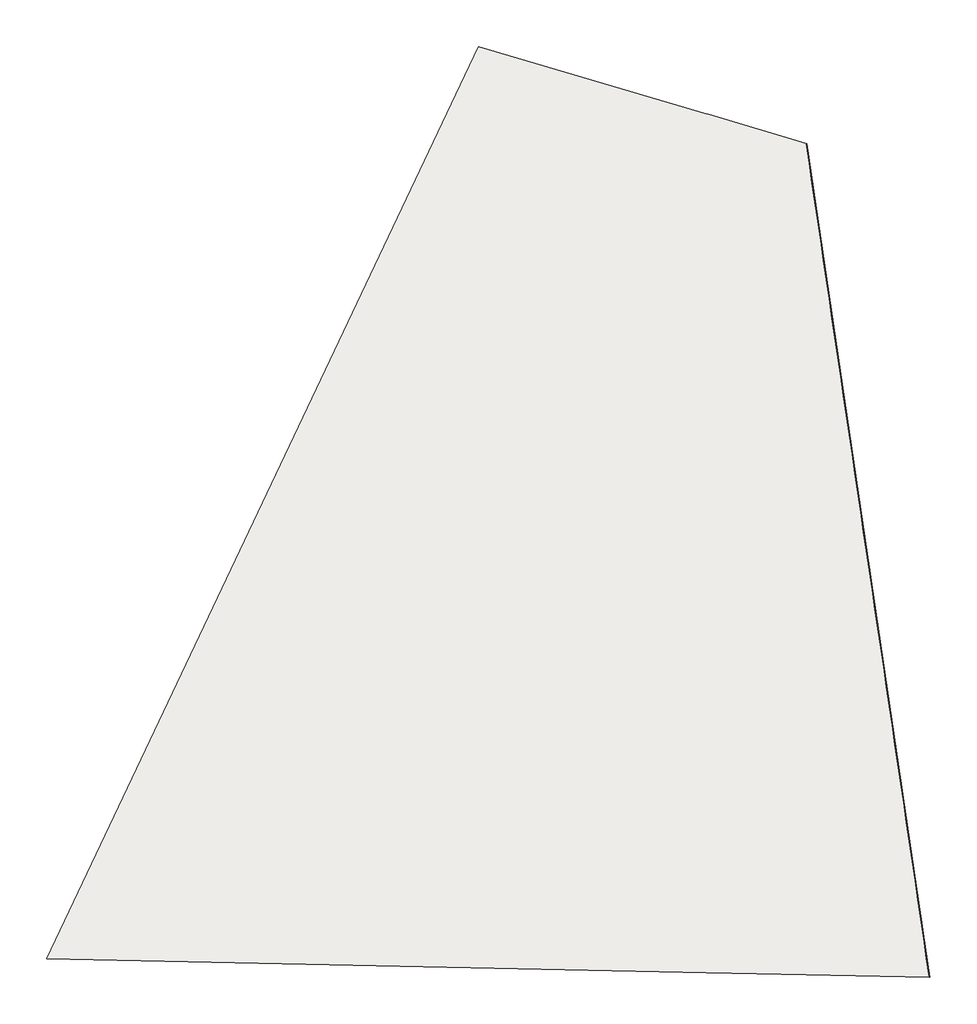
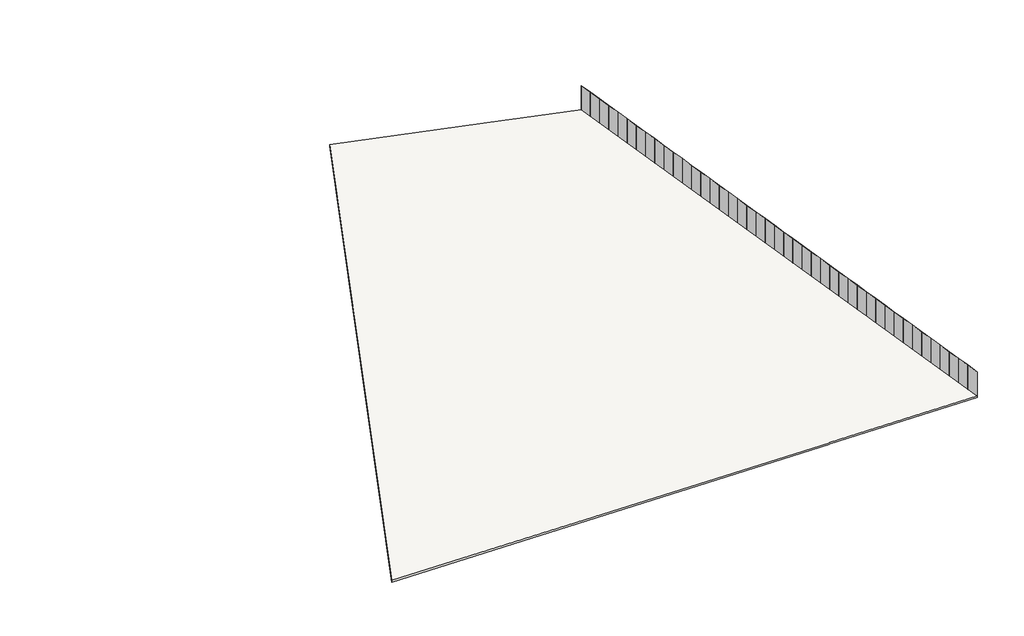
# One storey: 44 plates, 1 slab.
"""IFC4 building model written with IfcOpenShell, lengths in millimetres."""

import ifcopenshell
import ifcopenshell.guid

model = None  # the IFC model being written
_history = None  # IfcOwnerHistory: only IFC2X3 demands one
_inside = {}  # id of a spatial element -> (the spatial element, [elements in it])
_under = {}  # id of a project, library or spatial element -> (it, [spatial elements below it])
_declared = {}  # id of a project -> (the project, [libraries it declares])
_typed = {}  # id of a type object -> (the type object, [elements of that type])
_made_of = {}  # id of a material, layer set ... -> (it, [elements and type objects made of it])


def new_model(schema):
    """Start an empty IFC model of exactly this schema.

    Asked for "IFC4X3", IfcOpenShell would pick the latest addendum, in which some entities
    have other attributes; the version numbers below select the first issue.
    IFC2X3 requires an IfcOwnerHistory on every rooted entity: one is made here for all.
    """
    global model, _history
    if schema == "IFC4X3":
        model = ifcopenshell.file(schema_version=(4, 3, 0, 0))
    else:
        model = ifcopenshell.file(schema=schema)
    _inside.clear()
    _under.clear()
    _declared.clear()
    _typed.clear()
    _made_of.clear()
    _history = None
    if model.schema == "IFC2X3":
        org = make("IfcOrganization", Name="unknown")
        user = make(
            "IfcPersonAndOrganization",
            ThePerson=make("IfcPerson", FamilyName="unknown"),
            TheOrganization=org,
        )
        app = make(
            "IfcApplication",
            ApplicationDeveloper=org,
            Version="unknown",
            ApplicationFullName="unknown",
            ApplicationIdentifier="unknown",
        )
        _history = make(
            "IfcOwnerHistory",
            OwningUser=user,
            OwningApplication=app,
            ChangeAction="ADDED",
            CreationDate=0,
        )
    return model


def make(cls, **values):
    """One entity of the class cls with the attributes given. An attribute that is None is left unset."""
    return model.create_entity(
        cls, **{name: value for name, value in values.items() if value is not None}
    )


def rooted(cls, **values):
    """An entity with a GlobalId (a new one), such as an element, a storey or a relation."""
    return make(cls, GlobalId=ifcopenshell.guid.new(), OwnerHistory=_history, **values)


def si_unit(unit_type, name, prefix=None):
    """IfcSIUnit, for example si_unit("LENGTHUNIT", "METRE", prefix="MILLI")."""
    return make("IfcSIUnit", UnitType=unit_type, Prefix=prefix, Name=name)


def assignment(units):
    """IfcUnitAssignment: the units of a project."""
    return None if units is None else make("IfcUnitAssignment", Units=units)


def point(xyz):
    """IfcCartesianPoint."""
    return None if xyz is None else make("IfcCartesianPoint", Coordinates=xyz)


def direction(xyz):
    """IfcDirection."""
    return None if xyz is None else make("IfcDirection", DirectionRatios=xyz)


def frame(location, z_axis=None, x_axis=None):
    """IfcAxis2Placement3D, a coordinate frame: its origin and axes. An axis left out is left unset."""
    return make(
        "IfcAxis2Placement3D",
        Location=point(location),
        Axis=direction(z_axis),
        RefDirection=direction(x_axis),
    )


def origin():
    """The frame at (0, 0, 0) with its axes left unset."""
    return frame((0.0, 0.0, 0.0))


def origin_with_axes():
    """The frame at (0, 0, 0) with the z axis (0, 0, 1) and the x axis (1, 0, 0) written out."""
    return frame((0.0, 0.0, 0.0), z_axis=(0.0, 0.0, 1.0), x_axis=(1.0, 0.0, 0.0))


def place(relative_to, where):
    """IfcLocalPlacement: puts the frame where relative to a parent placement (None: the world)."""
    return make(
        "IfcLocalPlacement", PlacementRelTo=relative_to, RelativePlacement=where
    )


def context(
    kind, dimensions, precision=None, world=None, true_north=None, identifier=None
):
    """IfcGeometricRepresentationContext, for example the 3D "Model" context."""
    return make(
        "IfcGeometricRepresentationContext",
        ContextIdentifier=identifier,
        ContextType=kind,
        CoordinateSpaceDimension=dimensions,
        Precision=precision,
        WorldCoordinateSystem=world,
        TrueNorth=true_north,
    )


def project(units=None, contexts=None):
    """IfcProject with its units and contexts."""
    return rooted(
        "IfcProject",
        Name="project",
        RepresentationContexts=contexts,
        UnitsInContext=assignment(units),
    )


def spatial(cls, under=None, at=None, **own):
    """A site, building, storey or space (cls), placed at a placement, below another one or the project."""
    s = rooted(cls, ObjectPlacement=at, **own)
    if under is not None:
        _under.setdefault(under.id(), (under, []))[1].append(s)
    return s


def polyline(points):
    """IfcPolyline through the points."""
    return make("IfcPolyline", Points=[point(p) for p in points])


def outline(outer, holes=None, kind="AREA"):
    """IfcArbitraryClosedProfileDef: a profile drawn as a closed curve; with holes, ...WithVoids."""
    if holes is None:
        return make("IfcArbitraryClosedProfileDef", ProfileType=kind, OuterCurve=outer)
    return make(
        "IfcArbitraryProfileDefWithVoids",
        ProfileType=kind,
        OuterCurve=outer,
        InnerCurves=holes,
    )


def extrude(swept, where, along, depth):
    """IfcExtrudedAreaSolid: the profile swept, set in the frame where, extruded along a direction by depth."""
    return make(
        "IfcExtrudedAreaSolid",
        SweptArea=swept,
        Position=where,
        ExtrudedDirection=direction(along),
        Depth=depth,
    )


def faces_of(points, faces, orient=None, outer=None):
    """IfcFace entities. A face is a list of loops; a loop is a list of indices into points, from 0.

    orient and outer hold one flag for each loop. By default every Orientation is true, the
    first loop of a face is its IfcFaceOuterBound and the others are IfcFaceBound.
    """
    made = []
    for i, loops in enumerate(faces):
        bounds = []
        for j, loop in enumerate(loops):
            is_outer = j == 0 if outer is None else outer[i][j]
            bounds.append(
                make(
                    "IfcFaceOuterBound" if is_outer else "IfcFaceBound",
                    Bound=make("IfcPolyLoop", Polygon=[points[k] for k in loop]),
                    Orientation=True if orient is None else orient[i][j],
                )
            )
        made.append(make("IfcFace", Bounds=bounds))
    return made


def faceted_brep(points, faces, orient=None, outer=None, voids=None):
    """IfcFacetedBrep: a solid bounded by flat faces; with voids (closed shells), ...WithVoids."""
    shared = [point(p) for p in points]
    hull = make("IfcClosedShell", CfsFaces=faces_of(shared, faces, orient, outer))
    if voids is None:
        return make("IfcFacetedBrep", Outer=hull)
    return make(
        "IfcFacetedBrepWithVoids",
        Outer=hull,
        Voids=[
            make(cls, CfsFaces=faces_of(shared, fs, o, b)) for cls, fs, o, b in voids
        ],
    )


def shape(context_of_items, identifier, shape_type, items):
    """IfcShapeRepresentation: the items that make up one representation, for example the "Body"."""
    return make(
        "IfcShapeRepresentation",
        ContextOfItems=context_of_items,
        RepresentationIdentifier=identifier,
        RepresentationType=shape_type,
        Items=items,
    )


def source(mapping_origin, context_of_items, identifier, shape_type, items):
    """IfcRepresentationMap: a shape defined once, which mapped items show again and again."""
    return make(
        "IfcRepresentationMap",
        MappingOrigin=mapping_origin,
        MappedRepresentation=shape(context_of_items, identifier, shape_type, items),
    )


def transform(
    local_origin,
    x_axis=None,
    y_axis=None,
    z_axis=None,
    scale=None,
    scale2=None,
    scale3=None,
    uniform=True,
):
    """IfcCartesianTransformationOperator3D, or its non-uniform kind. x_axis, y_axis, z_axis: its Axis1, 2, 3."""
    if uniform:
        return make(
            "IfcCartesianTransformationOperator3D",
            Axis1=direction(x_axis),
            Axis2=direction(y_axis),
            LocalOrigin=point(local_origin),
            Scale=scale,
            Axis3=direction(z_axis),
        )
    return make(
        "IfcCartesianTransformationOperator3DnonUniform",
        Axis1=direction(x_axis),
        Axis2=direction(y_axis),
        LocalOrigin=point(local_origin),
        Scale=scale,
        Axis3=direction(z_axis),
        Scale2=scale2,
        Scale3=scale3,
    )


def mapped(mapping_source, mapping_target):
    """IfcMappedItem: shows the shape of a source again, moved by a transform."""
    return make(
        "IfcMappedItem", MappingSource=mapping_source, MappingTarget=mapping_target
    )


def made_of(thing, what):
    """Note that an element or type object is made of a material, layer set ...; save() writes the relation."""
    if what is not None:
        _made_of.setdefault(what.id(), (what, []))[1].append(thing)
    return thing


def element(
    cls,
    number,
    at=None,
    inside=None,
    cuts=None,
    type_object=None,
    material=None,
    context=None,
    identifier="Body",
    shape_type=None,
    held_by="IfcProductDefinitionShape",
    body=None,
    shapes=None,
    **own,
):
    """One element of the class cls, such as IfcWall. Its Tag is "e" and its number.

    at: its placement. inside: the storey or other place that contains it. cuts: it is an
    opening in that element (IfcRelVoidsElement). A single representation is given by context,
    identifier, shape_type and body (its items); several are given by shapes. held_by: the class
    of the entity that holds the representations. save() writes the other relations.
    """
    e = rooted(cls, Tag="e%d" % number, ObjectPlacement=at, **own)
    if body is not None:
        shapes = [shape(context, identifier, shape_type, body)]
    if shapes is not None:
        e.Representation = make(held_by, Representations=shapes)
    if inside is not None:
        _inside.setdefault(inside.id(), (inside, []))[1].append(e)
    if cuts is not None:
        rooted(
            "IfcRelVoidsElement", RelatingBuildingElement=cuts, RelatedOpeningElement=e
        )
    if type_object is not None:
        _typed.setdefault(type_object.id(), (type_object, []))[1].append(e)
    return made_of(e, material)


def aggregate(whole, parts):
    """IfcRelAggregates: a whole, such as a stair, and the parts it consists of."""
    return rooted("IfcRelAggregates", RelatingObject=whole, RelatedObjects=parts)


def save(model, path):
    """Write the relations noted so far, then the file.

    IfcRelAggregates (storeys below a building ...), IfcRelContainedInSpatialStructure (elements
    in a storey), IfcRelDefinesByType, IfcRelAssociatesMaterial and IfcRelDeclares: one each for
    every whole, place, type object, material and project.
    """
    for whole, parts in _under.values():
        aggregate(whole, parts)
    for where, things in _inside.values():
        rooted(
            "IfcRelContainedInSpatialStructure",
            RelatedElements=things,
            RelatingStructure=where,
        )
    for kind, things in _typed.values():
        rooted("IfcRelDefinesByType", RelatedObjects=things, RelatingType=kind)
    for what, things in _made_of.values():
        rooted("IfcRelAssociatesMaterial", RelatedObjects=things, RelatingMaterial=what)
    for by, libraries in _declared.values():
        rooted("IfcRelDeclares", RelatingContext=by, RelatedDefinitions=libraries)
    model.write(path)


def painel_do_sistema_b8becc76(model_context):
    return source(origin(), model_context, "Body", "SweptSolid", [
        extrude(outline(polyline([(1499.9999925, 24.5), (-1499.9999925, 24.5), (-1499.9999925, 49.5), (1499.9999925, 49.5), (1499.9999925, 24.5)])), origin_with_axes(), (0.0, 0.0, 1.0), 1500.0),
    ])


def painel_do_sistema_42adfd5d(model_context):
    return source(origin(), model_context, "Body", "SweptSolid", [
        extrude(outline(polyline([(1499.9999925, 24.5), (-1499.9999925, 24.5), (-1499.9999925, 49.5), (1499.9999925, 49.5), (1499.9999925, 24.5)])), origin_with_axes(), (0.0, 0.0, 1.0), 20.0931032),
    ])


model = new_model("IFC4")

# Units and contexts
model_context = context("Model", 3, world=origin())
ifc_project = project(units=[si_unit("LENGTHUNIT", "METRE", prefix="MILLI")], contexts=[model_context])

# Site, building, storey
site = spatial("IfcSite", under=ifc_project)
building = spatial("IfcBuilding", under=site)
storey = spatial("IfcBuildingStorey", under=building, Name="Nível 9", Elevation=12000.0)

# Plates
placement = place(None, origin())
painel_do_sistema_shape = painel_do_sistema_b8becc76(model_context)
element("IfcPlate", 1, ObjectType="Painel do sistema : Envidraçado", at=placement, inside=storey, context=model_context, shape_type="MappedRepresentation", body=[
    mapped(painel_do_sistema_shape, transform((27835.0106579, -36774.1442579, 13500.0000075), x_axis=(0.0, 0.0, 1.0), y_axis=(-0.9892699032546327, -0.1460994815684493, 0.0), z_axis=(0.1460994815684493, -0.9892699032546327, 0.0))),
])
element("IfcPlate", 2, ObjectType="Painel do sistema : Envidraçado", at=placement, inside=storey, context=model_context, shape_type="MappedRepresentation", body=[
    mapped(painel_do_sistema_shape, transform((27615.8614356, -35290.239403, 13500.0000075), x_axis=(0.0, 0.0, 1.0), y_axis=(-0.9892699032546328, -0.1460994815684489, 0.0), z_axis=(0.1460994815684489, -0.9892699032546328, 0.0))),
])
element("IfcPlate", 3, ObjectType="Painel do sistema : Envidraçado", at=placement, inside=storey, context=model_context, shape_type="MappedRepresentation", body=[
    mapped(painel_do_sistema_shape, transform((27396.7122132, -33806.3345481, 13500.0000075), x_axis=(0.0, 0.0, 1.0), y_axis=(-0.9892699032546323, -0.14609948156845212, 0.0), z_axis=(0.14609948156845212, -0.9892699032546323, 0.0))),
])
element("IfcPlate", 4, ObjectType="Painel do sistema : Envidraçado", at=placement, inside=storey, context=model_context, shape_type="MappedRepresentation", body=[
    mapped(painel_do_sistema_shape, transform((27177.5629909, -32322.4296932, 13500.0000075), x_axis=(0.0, 0.0, 1.0), y_axis=(-0.9892699032546327, -0.1460994815684493, 0.0), z_axis=(0.1460994815684493, -0.9892699032546327, 0.0))),
])
element("IfcPlate", 5, ObjectType="Painel do sistema : Envidraçado", at=placement, inside=storey, context=model_context, shape_type="MappedRepresentation", body=[
    mapped(painel_do_sistema_shape, transform((26958.4137685, -30838.5248383, 13500.0000075), x_axis=(0.0, 0.0, 1.0), y_axis=(-0.9892699032546327, -0.1460994815684493, 0.0), z_axis=(0.1460994815684493, -0.9892699032546327, 0.0))),
])
element("IfcPlate", 6, ObjectType="Painel do sistema : Envidraçado", at=placement, inside=storey, context=model_context, shape_type="MappedRepresentation", body=[
    mapped(painel_do_sistema_shape, transform((26739.2645462, -29354.6199835, 13500.0000075), x_axis=(0.0, 0.0, 1.0), y_axis=(-0.9892699032546327, -0.1460994815684493, 0.0), z_axis=(0.1460994815684493, -0.9892699032546327, 0.0))),
])
element("IfcPlate", 7, ObjectType="Painel do sistema : Envidraçado", at=placement, inside=storey, context=model_context, shape_type="MappedRepresentation", body=[
    mapped(painel_do_sistema_shape, transform((26520.1153238, -27870.7151286, 13500.0000075), x_axis=(0.0, 0.0, 1.0), y_axis=(-0.9892699032546324, -0.14609948156845168, 0.0), z_axis=(0.14609948156845168, -0.9892699032546324, 0.0))),
])
element("IfcPlate", 8, ObjectType="Painel do sistema : Envidraçado", at=placement, inside=storey, context=model_context, shape_type="MappedRepresentation", body=[
    mapped(painel_do_sistema_shape, transform((26300.9661014, -26386.8102737, 13500.0000075), x_axis=(0.0, 0.0, 1.0), y_axis=(-0.9892699032546327, -0.1460994815684493, 0.0), z_axis=(0.1460994815684493, -0.9892699032546327, 0.0))),
])
element("IfcPlate", 9, ObjectType="Painel do sistema : Envidraçado", at=placement, inside=storey, context=model_context, shape_type="MappedRepresentation", body=[
    mapped(painel_do_sistema_shape, transform((26081.8168791, -24902.9054188, 13500.0000075), x_axis=(0.0, 0.0, 1.0), y_axis=(-0.9892699032546328, -0.1460994815684489, 0.0), z_axis=(0.1460994815684489, -0.9892699032546328, 0.0))),
])
element("IfcPlate", 10, ObjectType="Painel do sistema : Envidraçado", at=placement, inside=storey, context=model_context, shape_type="MappedRepresentation", body=[
    mapped(painel_do_sistema_shape, transform((25862.6676567, -23419.0005639, 13500.0000075), x_axis=(0.0, 0.0, 1.0), y_axis=(-0.9892699032546324, -0.14609948156845168, 0.0), z_axis=(0.14609948156845168, -0.9892699032546324, 0.0))),
])
element("IfcPlate", 11, ObjectType="Painel do sistema : Envidraçado", at=placement, inside=storey, context=model_context, shape_type="MappedRepresentation", body=[
    mapped(painel_do_sistema_shape, transform((25643.5184344, -21935.095709, 13500.0000075), x_axis=(0.0, 0.0, 1.0), y_axis=(-0.9892699032546327, -0.1460994815684493, 0.0), z_axis=(0.1460994815684493, -0.9892699032546327, 0.0))),
])
element("IfcPlate", 12, ObjectType="Painel do sistema : Envidraçado", at=placement, inside=storey, context=model_context, shape_type="MappedRepresentation", body=[
    mapped(painel_do_sistema_shape, transform((25424.369212, -20451.1908542, 13500.0000075), x_axis=(0.0, 0.0, 1.0), y_axis=(-0.9892699032546324, -0.14609948156845168, 0.0), z_axis=(0.14609948156845168, -0.9892699032546324, 0.0))),
])
element("IfcPlate", 13, ObjectType="Painel do sistema : Envidraçado", at=placement, inside=storey, context=model_context, shape_type="MappedRepresentation", body=[
    mapped(painel_do_sistema_shape, transform((25205.2199897, -18967.2859993, 13500.0000075), x_axis=(0.0, 0.0, 1.0), y_axis=(-0.9892699032546328, -0.14609948156844865, 0.0), z_axis=(0.14609948156844865, -0.9892699032546328, 0.0))),
])
element("IfcPlate", 14, ObjectType="Painel do sistema : Envidraçado", at=placement, inside=storey, context=model_context, shape_type="MappedRepresentation", body=[
    mapped(painel_do_sistema_shape, transform((24986.0707673, -17483.3811444, 13500.0000075), x_axis=(0.0, 0.0, 1.0), y_axis=(-0.9892699032546328, -0.1460994815684491, 0.0), z_axis=(0.1460994815684491, -0.9892699032546328, 0.0))),
])
element("IfcPlate", 15, ObjectType="Painel do sistema : Envidraçado", at=placement, inside=storey, context=model_context, shape_type="MappedRepresentation", body=[
    mapped(painel_do_sistema_shape, transform((24766.921545, -15999.4762895, 13500.0000075), x_axis=(0.0, 0.0, 1.0), y_axis=(-0.9892699032546327, -0.1460994815684493, 0.0), z_axis=(0.1460994815684493, -0.9892699032546327, 0.0))),
])
element("IfcPlate", 16, ObjectType="Painel do sistema : Envidraçado", at=placement, inside=storey, context=model_context, shape_type="MappedRepresentation", body=[
    mapped(painel_do_sistema_shape, transform((24547.7723226, -14515.5714346, 13500.0000075), x_axis=(0.0, 0.0, 1.0), y_axis=(-0.9892699032546324, -0.14609948156845168, 0.0), z_axis=(0.14609948156845168, -0.9892699032546324, 0.0))),
])
element("IfcPlate", 17, ObjectType="Painel do sistema : Envidraçado", at=placement, inside=storey, context=model_context, shape_type="MappedRepresentation", body=[
    mapped(painel_do_sistema_shape, transform((24328.6231003, -13031.6665798, 13500.0000075), x_axis=(0.0, 0.0, 1.0), y_axis=(-0.9892699032546327, -0.14609948156844949, 0.0), z_axis=(0.14609948156844949, -0.9892699032546327, 0.0))),
])
element("IfcPlate", 18, ObjectType="Painel do sistema : Envidraçado", at=placement, inside=storey, context=model_context, shape_type="MappedRepresentation", body=[
    mapped(painel_do_sistema_shape, transform((24109.4738779, -11547.7617249, 13500.0000075), x_axis=(0.0, 0.0, 1.0), y_axis=(-0.9892699032546328, -0.1460994815684491, 0.0), z_axis=(0.1460994815684491, -0.9892699032546328, 0.0))),
])
element("IfcPlate", 19, ObjectType="Painel do sistema : Envidraçado", at=placement, inside=storey, context=model_context, shape_type="MappedRepresentation", body=[
    mapped(painel_do_sistema_shape, transform((23890.3246556, -10063.85687, 13500.0000075), x_axis=(0.0, 0.0, 1.0), y_axis=(-0.9892699032546325, -0.14609948156845148, 0.0), z_axis=(0.14609948156845148, -0.9892699032546325, 0.0))),
])
element("IfcPlate", 20, ObjectType="Painel do sistema : Envidraçado", at=placement, inside=storey, context=model_context, shape_type="MappedRepresentation", body=[
    mapped(painel_do_sistema_shape, transform((23671.1754332, -8579.9520151, 13500.0000075), x_axis=(0.0, 0.0, 1.0), y_axis=(-0.9892699032546332, -0.14609948156844624, 0.0), z_axis=(0.14609948156844624, -0.9892699032546332, 0.0))),
])
element("IfcPlate", 21, ObjectType="Painel do sistema : Envidraçado", at=placement, inside=storey, context=model_context, shape_type="MappedRepresentation", body=[
    mapped(painel_do_sistema_shape, transform((23452.0262109, -7096.0471602, 13500.0000075), x_axis=(0.0, 0.0, 1.0), y_axis=(-0.9892699032546319, -0.14609948156845476, 0.0), z_axis=(0.14609948156845476, -0.9892699032546319, 0.0))),
])
element("IfcPlate", 22, ObjectType="Painel do sistema : Envidraçado", at=placement, inside=storey, context=model_context, shape_type="MappedRepresentation", body=[
    mapped(painel_do_sistema_shape, transform((23232.8769885, -5612.1423053, 13500.0000075), x_axis=(0.0, 0.0, 1.0), y_axis=(-0.9892699032546332, -0.14609948156844646, 0.0), z_axis=(0.14609948156844646, -0.9892699032546332, 0.0))),
])
element("IfcPlate", 23, ObjectType="Painel do sistema : Envidraçado", at=placement, inside=storey, context=model_context, shape_type="MappedRepresentation", body=[
    mapped(painel_do_sistema_shape, transform((23013.7277662, -4128.2374505, 13500.0000075), x_axis=(0.0, 0.0, 1.0), y_axis=(-0.9892699032546324, -0.14609948156845168, 0.0), z_axis=(0.14609948156845168, -0.9892699032546324, 0.0))),
])
element("IfcPlate", 24, ObjectType="Painel do sistema : Envidraçado", at=placement, inside=storey, context=model_context, shape_type="MappedRepresentation", body=[
    mapped(painel_do_sistema_shape, transform((22794.5785438, -2644.3325956, 13500.0000075), x_axis=(0.0, 0.0, 1.0), y_axis=(-0.9892699032546329, -0.14609948156844868, 0.0), z_axis=(0.14609948156844868, -0.9892699032546329, 0.0))),
])
element("IfcPlate", 25, ObjectType="Painel do sistema : Envidraçado", at=placement, inside=storey, context=model_context, shape_type="MappedRepresentation", body=[
    mapped(painel_do_sistema_shape, transform((22575.4293215, -1160.4277407, 13500.0000075), x_axis=(0.0, 0.0, 1.0), y_axis=(-0.9892699032546327, -0.1460994815684493, 0.0), z_axis=(0.1460994815684493, -0.9892699032546327, 0.0))),
])
element("IfcPlate", 26, ObjectType="Painel do sistema : Envidraçado", at=placement, inside=storey, context=model_context, shape_type="MappedRepresentation", body=[
    mapped(painel_do_sistema_shape, transform((22356.2800991, 323.4771142, 13500.0000075), x_axis=(0.0, 0.0, 1.0), y_axis=(-0.9892699032546325, -0.14609948156845148, 0.0), z_axis=(0.14609948156845148, -0.9892699032546325, 0.0))),
])
element("IfcPlate", 27, ObjectType="Painel do sistema : Envidraçado", at=placement, inside=storey, context=model_context, shape_type="MappedRepresentation", body=[
    mapped(painel_do_sistema_shape, transform((22137.1308767, 1807.3819691, 13500.0000075), x_axis=(0.0, 0.0, 1.0), y_axis=(-0.9892699032546332, -0.14609948156844688, 0.0), z_axis=(0.14609948156844688, -0.9892699032546332, 0.0))),
])
element("IfcPlate", 28, ObjectType="Painel do sistema : Envidraçado", at=placement, inside=storey, context=model_context, shape_type="MappedRepresentation", body=[
    mapped(painel_do_sistema_shape, transform((21917.9816544, 3291.2868239, 13500.0000075), x_axis=(0.0, 0.0, 1.0), y_axis=(-0.9892699032546323, -0.1460994815684521, 0.0), z_axis=(0.1460994815684521, -0.9892699032546323, 0.0))),
])
element("IfcPlate", 29, ObjectType="Painel do sistema : Envidraçado", at=placement, inside=storey, context=model_context, shape_type="MappedRepresentation", body=[
    mapped(painel_do_sistema_shape, transform((21698.832432, 4775.1916788, 13500.0000075), x_axis=(0.0, 0.0, 1.0), y_axis=(-0.9892699032546323, -0.14609948156845232, 0.0), z_axis=(0.14609948156845232, -0.9892699032546323, 0.0))),
])
element("IfcPlate", 30, ObjectType="Painel do sistema : Envidraçado", at=placement, inside=storey, context=model_context, shape_type="MappedRepresentation", body=[
    mapped(painel_do_sistema_shape, transform((21479.6832097, 6259.0965337, 13500.0000075), x_axis=(0.0, 0.0, 1.0), y_axis=(-0.9892699032546332, -0.14609948156844646, 0.0), z_axis=(0.14609948156844646, -0.9892699032546332, 0.0))),
])
element("IfcPlate", 31, ObjectType="Painel do sistema : Envidraçado", at=placement, inside=storey, context=model_context, shape_type="MappedRepresentation", body=[
    mapped(painel_do_sistema_shape, transform((21260.5339873, 7743.0013886, 13500.0000075), x_axis=(0.0, 0.0, 1.0), y_axis=(-0.9892699032546323, -0.14609948156845232, 0.0), z_axis=(0.14609948156845232, -0.9892699032546323, 0.0))),
])
element("IfcPlate", 32, ObjectType="Painel do sistema : Envidraçado", at=placement, inside=storey, context=model_context, shape_type="MappedRepresentation", body=[
    mapped(painel_do_sistema_shape, transform((21041.384765, 9226.9062435, 13500.0000075), x_axis=(0.0, 0.0, 1.0), y_axis=(-0.9892699032546327, -0.14609948156844949, 0.0), z_axis=(0.14609948156844949, -0.9892699032546327, 0.0))),
])
element("IfcPlate", 33, ObjectType="Painel do sistema : Envidraçado", at=placement, inside=storey, context=model_context, shape_type="MappedRepresentation", body=[
    mapped(painel_do_sistema_shape, transform((20822.2355426, 10710.8110984, 13500.0000075), x_axis=(0.0, 0.0, 1.0), y_axis=(-0.9892699032546327, -0.14609948156844949, 0.0), z_axis=(0.14609948156844949, -0.9892699032546327, 0.0))),
])
element("IfcPlate", 34, ObjectType="Painel do sistema : Envidraçado", at=placement, inside=storey, context=model_context, shape_type="MappedRepresentation", body=[
    mapped(painel_do_sistema_shape, transform((20603.0863203, 12194.7159532, 13500.0000075), x_axis=(0.0, 0.0, 1.0), y_axis=(-0.9892699032546327, -0.14609948156844949, 0.0), z_axis=(0.14609948156844949, -0.9892699032546327, 0.0))),
])
element("IfcPlate", 35, ObjectType="Painel do sistema : Envidraçado", at=placement, inside=storey, context=model_context, shape_type="MappedRepresentation", body=[
    mapped(painel_do_sistema_shape, transform((20383.9370979, 13678.6208081, 13500.0000075), x_axis=(0.0, 0.0, 1.0), y_axis=(-0.9892699032546325, -0.1460994815684505, 0.0), z_axis=(0.1460994815684505, -0.9892699032546325, 0.0))),
])
element("IfcPlate", 36, ObjectType="Painel do sistema : Envidraçado", at=placement, inside=storey, context=model_context, shape_type="MappedRepresentation", body=[
    mapped(painel_do_sistema_shape, transform((20164.7878756, 15162.525663, 13500.0000075), x_axis=(0.0, 0.0, 1.0), y_axis=(-0.9892699032546328, -0.14609948156844887, 0.0), z_axis=(0.14609948156844887, -0.9892699032546328, 0.0))),
])
element("IfcPlate", 37, ObjectType="Painel do sistema : Envidraçado", at=placement, inside=storey, context=model_context, shape_type="MappedRepresentation", body=[
    mapped(painel_do_sistema_shape, transform((19945.6386532, 16646.4305179, 13500.0000075), x_axis=(0.0, 0.0, 1.0), y_axis=(-0.9892699032546327, -0.1460994815684493, 0.0), z_axis=(0.1460994815684493, -0.9892699032546327, 0.0))),
])
element("IfcPlate", 38, ObjectType="Painel do sistema : Envidraçado", at=placement, inside=storey, context=model_context, shape_type="MappedRepresentation", body=[
    mapped(painel_do_sistema_shape, transform((19726.4894309, 18130.3353728, 13500.0000075), x_axis=(0.0, 0.0, 1.0), y_axis=(-0.9892699032546327, -0.14609948156845012, 0.0), z_axis=(0.14609948156845012, -0.9892699032546327, 0.0))),
])
element("IfcPlate", 39, ObjectType="Painel do sistema : Envidraçado", at=placement, inside=storey, context=model_context, shape_type="MappedRepresentation", body=[
    mapped(painel_do_sistema_shape, transform((19507.3402085, 19614.2402276, 13500.0000075), x_axis=(0.0, 0.0, 1.0), y_axis=(-0.9892699032546329, -0.14609948156844846, 0.0), z_axis=(0.14609948156844846, -0.9892699032546329, 0.0))),
])
element("IfcPlate", 40, ObjectType="Painel do sistema : Envidraçado", at=placement, inside=storey, context=model_context, shape_type="MappedRepresentation", body=[
    mapped(painel_do_sistema_shape, transform((19288.1909862, 21098.1450825, 13500.0000075), x_axis=(0.0, 0.0, 1.0), y_axis=(-0.9892699032546323, -0.14609948156845254, 0.0), z_axis=(0.14609948156845254, -0.9892699032546323, 0.0))),
])
element("IfcPlate", 41, ObjectType="Painel do sistema : Envidraçado", at=placement, inside=storey, context=model_context, shape_type="MappedRepresentation", body=[
    mapped(painel_do_sistema_shape, transform((19069.0417638, 22582.0499374, 13500.0000075), x_axis=(0.0, 0.0, 1.0), y_axis=(-0.9892699032546327, -0.1460994815684497, 0.0), z_axis=(0.1460994815684497, -0.9892699032546327, 0.0))),
])
element("IfcPlate", 42, ObjectType="Painel do sistema : Envidraçado", at=placement, inside=storey, context=model_context, shape_type="MappedRepresentation", body=[
    mapped(painel_do_sistema_shape, transform((18849.8925415, 24065.9547923, 13500.0000075), x_axis=(0.0, 0.0, 1.0), y_axis=(-0.9892699032546327, -0.14609948156845012, 0.0), z_axis=(0.14609948156845012, -0.9892699032546327, 0.0))),
])
element("IfcPlate", 43, ObjectType="Painel do sistema : Envidraçado", at=placement, inside=storey, context=model_context, shape_type="MappedRepresentation", body=[
    mapped(painel_do_sistema_shape, transform((18630.7433191, 25549.8596472, 13500.0000075), x_axis=(0.0, 0.0, 1.0), y_axis=(-0.9892699032546326, -0.14609948156844987, 0.0), z_axis=(0.14609948156844987, -0.9892699032546326, 0.0))),
])
painel_do_sistema_2_shape = painel_do_sistema_42adfd5d(model_context)
element("IfcPlate", 44, ObjectType="Painel do sistema : Envidraçado", at=placement, inside=storey, context=model_context, shape_type="MappedRepresentation", body=[
    mapped(painel_do_sistema_2_shape, transform((18627.8077271, 25569.7371494, 13500.0000075), x_axis=(0.0, 0.0, 1.0), y_axis=(-0.9892699032546368, -0.14609948156842112, 0.0), z_axis=(0.14609948156842112, -0.9892699032546368, 0.0))),
])

# Slab
element("IfcSlab", 45, ObjectType="piso aula 04", at=placement, inside=storey, context=model_context, shape_type="Brep", body=[
    faceted_brep([(18627.8077271, 25569.7371494, 11790.0), (28054.1598803, -38258.0491127, 11790.0), (10995.3657537, -37899.7374539, 11790.0), (10920.3657537, -37898.1621155, 11790.0), (-39610.4993669, -36836.7859146, 11790.0), (-6526.0277886, 32996.9225357, 11790.0), (10995.3657537, 27823.3720454, 11790.0), (11070.3657537, 27801.2267585, 11790.0), (18627.8077271, 25569.7371494, 12000.0), (11070.3657537, 27801.2267585, 12000.0), (10995.3657537, 27823.3720454, 12000.0), (-6526.0277886, 32996.9225357, 12000.0), (-39610.4993669, -36836.7859146, 12000.0), (10920.3657537, -37898.1621155, 12000.0), (10995.3657537, -37899.7374539, 12000.0), (28054.1598803, -38258.0491127, 12000.0)], [[[0, 1, 2, 3, 4, 5, 6, 7]], [[8, 9, 10, 11, 12, 13, 14, 15]], [[1, 0, 8, 15]], [[4, 3, 2, 1, 15, 14, 13, 12]], [[5, 4, 12, 11]], [[0, 7, 6, 5, 11, 10, 9, 8]]]),
])

save(model, "model.ifc")

# Revit data of these elements
# Type "Painel do sistema : Envidraçado"
#   Construction Type Id = "GSP4R"
#   Analytic Construction = "Vidraça única Pilkington 1/8 pol"
#   Visual Light Transmittance = 0.9
#   Solar Heat Gain Coefficient = 0.86
#   Heat Transfer Coefficient (U) = 6.7069 W/(m²·K)
# Type "piso aula 04"
#   Function = 0
#   Layers, outside or top first: 0.02 m "Azulejo cerâmico" (function 4); 0.04 m "Concreto, Faixa de areia/cimento" (function 2); 0.15 m "Concreto,  Moldado in loco" (function 1)
# Elements 1, 2, 3, 4, 5, 6, 7, 8, 9, 10, 11, 12, 13, 14, 15, 16, 17, 18, 19, 20, 21, 22, 23, 24, 25, 26, 27, 28, 29, 30, 31, 32, 33, 34, 35, 36, 37, 38, 39, 40, 41, 42, 43, 44 (IfcPlate, "Painel do sistema : Envidraçado")
#   Phase Created = Construção nova
#   Materials on its faces: "Vidro"
# Element 45 (IfcSlab, "piso aula 04")
#   built-in parameter 1001955 = -0.287112 (stored number, unit not read)
#   Height Offset From Level = 0.00 m
#   Phase Created = Construção nova
#   Materials on its faces: "Concreto,  Moldado in loco", "Azulejo cerâmico"
# Materials
#   "Azulejo cerâmico": class "Cerâmica", colour RGB 246 230 196, transparency 0, Description = "Material físico", Cost = 0
#   "Concreto, Faixa de areia/cimento": class "Concreto", colour RGB 127 127 127, transparency 0, Description = "Revestimento de laje de concreto", Cost = 0
#   "Concreto,  Moldado in loco": class "Concreto", colour RGB 192 192 192, transparency 0, Description = "Material físico", Cost = 0
#   "Vidro": class "Vidro", colour RGB 0 128 192, transparency 0.9, Description = "Vidro de sílica", Cost = 0
